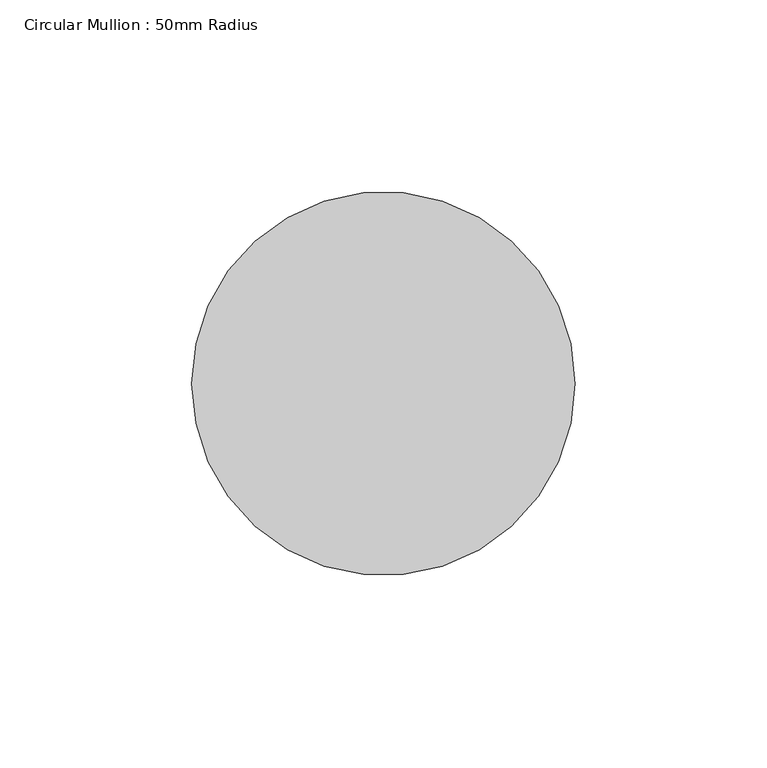
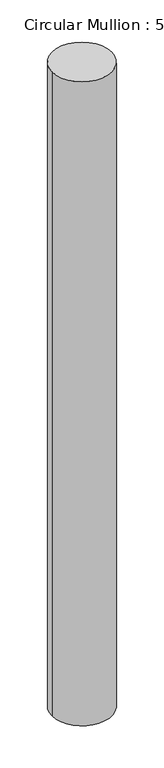
"""IFC4 building model written with IfcOpenShell, lengths in millimetres: member geometry, Circular Mullion : 50mm Radius."""

from ifc_helpers import new_model, si_unit, point, frame, origin, origin_2d, place, context, project, spatial, circle_curve, trimmed, segment, composite_curve, outline, extrude, source, transform, mapped, element, save


def circular_mullion_50mm_radius_ec59be0d(model_context):
    return source(origin(), model_context, "Body", "SweptSolid", [
        extrude(outline(composite_curve([segment(trimmed(circle_curve(origin_2d(), 50.0), [point((50.0, 0.0))], [point((-50.0, 0.0))], False, "CARTESIAN"), True, "CONTINUOUS"), segment(trimmed(circle_curve(origin_2d(), 50.0), [point((-50.0, 0.0))], [point((50.0, 0.0))], False, "CARTESIAN"), True, "CONTINUOUS")], self_intersect=False)), frame((0.0, 0.0, -1137.5257799), z_axis=(0.0, 0.0, 1.0), x_axis=(1.0, 0.0, 0.0)), (0.0, 0.0, 1.0), 1137.5257799),
    ])


if __name__ == "__main__":
    model = new_model("IFC4")
    model_context = context("Model", 3, world=origin())
    ifc_project = project(units=[si_unit("LENGTHUNIT", "METRE", prefix="MILLI")], contexts=[model_context])
    site = spatial("IfcSite", under=ifc_project)
    building = spatial("IfcBuilding", under=site)
    placement = place(None, origin())
    circular_mullion_50mm_radius_shape = circular_mullion_50mm_radius_ec59be0d(model_context)
    element("IfcMember", 1, ObjectType="Circular Mullion : 50mm Radius", at=placement, inside=building, context=model_context, shape_type="MappedRepresentation", body=[
        mapped(circular_mullion_50mm_radius_shape, transform((0.0, 0.0, 0.0), x_axis=(1.0, 0.0, 0.0), y_axis=(0.0, 1.0, 0.0), z_axis=(0.0, 0.0, 1.0))),
    ])
    save(model, "model.ifc")

# Revit data of these elements
# Type "Circular Mullion : 50mm Radius"
#   built-in parameter 1007350 = 0.164042 (stored number, unit not read)
# Element 1 (IfcMember, "Circular Mullion : 50mm Radius")
#   Materials on its faces: "Aluminium"
# Materials
#   "Aluminium": class "Metal", colour RGB 247 247 247, transparency 0, Description = "Aluminium 6061", Cost = 0
